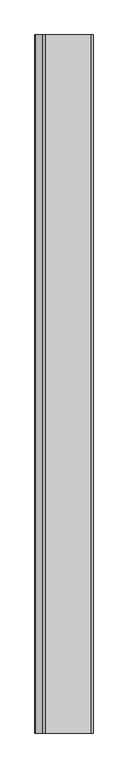
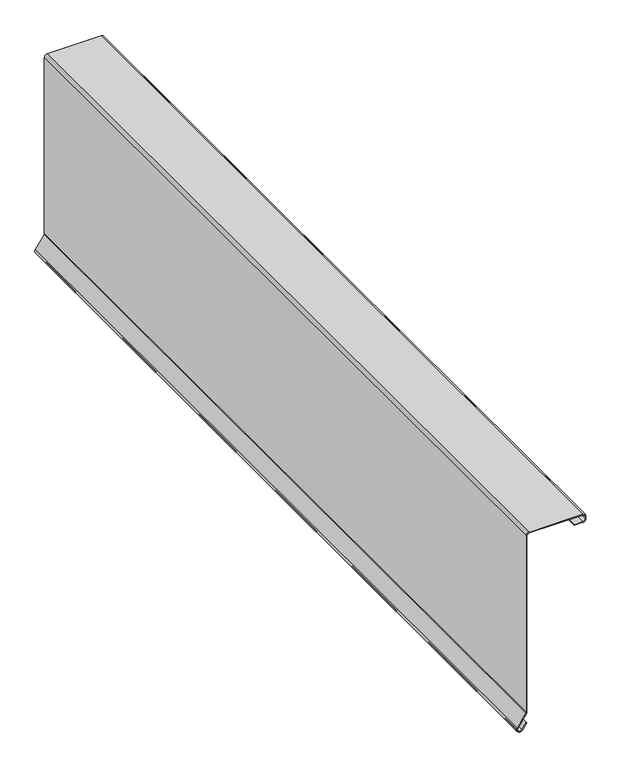
"""IFC4 building model written with IfcOpenShell, lengths in millimetres: proxy geometry, Flashing16:Flashing012:299211 : Flashing16:Flashing012:299211."""

from ifc_helpers import new_model, si_unit, point, frame, frame_2d, origin, place, context, project, spatial, polyline, circle_curve, trimmed, segment, composite_curve, outline, extrude, source, transform, mapped, element, save


def generic_models_2aed0af1(model_context):
    return source(origin(), model_context, "Body", "SweptSolid", [
        extrude(outline(composite_curve([segment(polyline([(42123.2180833, 2308.4687491), (42108.6312101, 2298.2115016)]), True, "CONTINUOUS"), segment(trimmed(circle_curve(frame_2d((42111.5532705, 2294.0560278)), 5.08), [point((42108.6312101, 2298.2115016))], [point((42107.4417652, 2291.0724184))], True, "CARTESIAN"), True, "CONTINUOUS"), segment(polyline([(42107.4417652, 2291.0724184), (42108.7344443, 2289.291067)]), True, "CONTINUOUS"), segment(trimmed(circle_curve(frame_2d((42112.8459496, 2292.2746763)), 5.08), [point((42108.7344443, 2289.291067))], [point((42115.753039, 2288.1087153))], True, "CARTESIAN"), True, "CONTINUOUS"), segment(polyline([(42115.753039, 2288.1087153), (42146.0058896, 2309.2197491)]), True, "CONTINUOUS"), segment(trimmed(circle_curve(frame_2d((42148.9129791, 2305.0537881)), 5.08), [point((42146.0058896, 2309.2197491))], [point((42148.9129791, 2310.1337881))], False, "CARTESIAN"), True, "CONTINUOUS"), segment(polyline([(42148.9129791, 2310.1337881), (42596.1419896, 2310.1337881)]), True, "CONTINUOUS"), segment(trimmed(circle_curve(frame_2d((42596.1419896, 2315.2137881)), 5.08), [point((42596.1419896, 2310.1337881))], [point((42601.2219896, 2315.2137881))], True, "CARTESIAN"), True, "CONTINUOUS"), segment(polyline([(42601.2219896, 2315.2137881), (42601.2219896, 2444.5537881)]), True, "CONTINUOUS"), segment(trimmed(circle_curve(frame_2d((42596.1419896, 2444.5537881)), 5.08), [point((42601.2219896, 2444.5537881))], [point((42596.1419896, 2449.6337881))], True, "CARTESIAN"), True, "CONTINUOUS"), segment(polyline([(42596.1419896, 2449.6337881), (42589.7355833, 2449.6337881)]), True, "CONTINUOUS"), segment(trimmed(circle_curve(frame_2d((42589.7355833, 2444.5537881)), 5.08), [point((42589.7355833, 2449.6337881))], [point((42584.6555833, 2444.5537881))], True, "CARTESIAN"), True, "CONTINUOUS"), segment(polyline([(42584.6555833, 2444.5537881), (42584.6555833, 2423.2573233), (42582.6555833, 2423.2573233), (42582.6555833, 2444.5537881)]), True, "CONTINUOUS"), segment(trimmed(circle_curve(frame_2d((42589.7355833, 2444.5537881)), 7.08), [point((42582.6555833, 2444.5537881))], [point((42589.7355833, 2451.6337881))], False, "CARTESIAN"), True, "CONTINUOUS"), segment(polyline([(42589.7355833, 2451.6337881), (42596.1419896, 2451.6337881)]), True, "CONTINUOUS"), segment(trimmed(circle_curve(frame_2d((42596.1419896, 2444.5537881)), 7.08), [point((42596.1419896, 2451.6337881))], [point((42603.2219896, 2444.5537881))], False, "CARTESIAN"), True, "CONTINUOUS"), segment(polyline([(42603.2219896, 2444.5537881), (42603.2219896, 2315.2137881)]), True, "CONTINUOUS"), segment(trimmed(circle_curve(frame_2d((42596.1419896, 2315.2137881)), 7.08), [point((42603.2219896, 2315.2137881))], [point((42596.1419896, 2308.1337881))], False, "CARTESIAN"), True, "CONTINUOUS"), segment(polyline([(42596.1419896, 2308.1337881), (42148.9129791, 2308.1337881)]), True, "CONTINUOUS"), segment(trimmed(circle_curve(frame_2d((42148.9129791, 2305.0537881)), 3.08), [point((42148.9129791, 2308.1337881))], [point((42147.150413, 2307.579607))], True, "CARTESIAN"), True, "CONTINUOUS"), segment(polyline([(42147.150413, 2307.579607), (42116.8975624, 2286.4685732)]), True, "CONTINUOUS"), segment(trimmed(circle_curve(frame_2d((42112.8459496, 2292.2746763)), 7.08), [point((42116.8975624, 2286.4685732))], [point((42107.1157415, 2288.1164176))], False, "CARTESIAN"), True, "CONTINUOUS"), segment(polyline([(42107.1157415, 2288.1164176), (42105.8230624, 2289.8977691)]), True, "CONTINUOUS"), segment(trimmed(circle_curve(frame_2d((42111.5532705, 2294.0560278)), 7.08), [point((42105.8230624, 2289.8977691))], [point((42107.4807927, 2299.847515))], False, "CARTESIAN"), True, "CONTINUOUS"), segment(polyline([(42107.4807927, 2299.847515), (42122.0676658, 2310.1047624), (42123.2180833, 2308.4687491)]), True, "CONTINUOUS")], self_intersect=False)), frame((0.0, -774.5581163, 0.0), z_axis=(0.0, 1.0, 0.0), x_axis=(0.0, 0.0, 1.0)), (0.0, 0.0, 1.0), 2000.0),
    ])


if __name__ == "__main__":
    model = new_model("IFC4")
    model_context = context("Model", 3, world=origin())
    ifc_project = project(units=[si_unit("LENGTHUNIT", "METRE", prefix="MILLI")], contexts=[model_context])
    site = spatial("IfcSite", under=ifc_project)
    building = spatial("IfcBuilding", under=site)
    placement = place(None, origin())
    generic_models_shape = generic_models_2aed0af1(model_context)
    element("IfcBuildingElementProxy", 1, Name="Flashing16:Flashing012:299211 : Flashing16:Flashing012:299211", ObjectType="Flashing16:Flashing012:299211 : Flashing16:Flashing012:299211", at=placement, inside=building, context=model_context, shape_type="MappedRepresentation", body=[
        mapped(generic_models_shape, transform((0.0, 0.0, 0.0), x_axis=(1.0, 0.0, 0.0), y_axis=(0.0, 1.0, 0.0), z_axis=(0.0, 0.0, 1.0))),
    ])
    save(model, "model.ifc")

# Revit data of these elements
# Type "Flashing16:Flashing012:299211 : Flashing16:Flashing012:299211"
#   NameOverride = "Flashing16:Flashing012:299211"
#   ObjectTypeOverride = "Flashing16:Flashing012"
#   Reference = "Flashing012"
#   Category = "Generic Models"
#   Tag = "299211"
# Element 1 (IfcBuildingElementProxy, "Flashing16:Flashing012:299211 : Flashing16:Flashing012:299211")
#   Materials on its faces: "HIGH EAVE FLASHING"
# Materials
#   "HIGH EAVE FLASHING": class "Unassigned", colour RGB 128 128 128, transparency 0, Cost = 0
